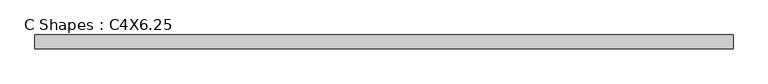
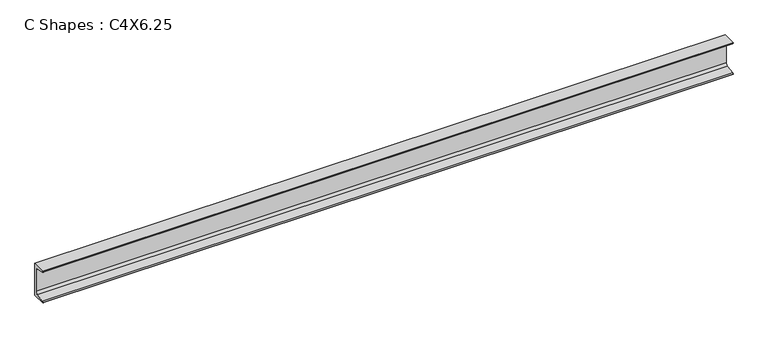
"""IFC4 building model written with IfcOpenShell, lengths in millimetres: beam geometry, C Shapes : C4X6.25."""

from ifc_helpers import new_model, si_unit, point, frame, frame_2d, origin, place, context, project, spatial, polyline, circle_curve, trimmed, segment, composite_curve, outline, extrude, source, transform, mapped, element, save


def c_shapes_c4x6_25_9ff4ea91(model_context):
    return source(origin(), model_context, "Body", "SweptSolid", [
        extrude(outline(composite_curve([segment(polyline([(11.049, 50.8), (11.049, -50.8), (-30.861, -50.8), (-30.861, -49.7865772)]), True, "CONTINUOUS"), segment(trimmed(circle_curve(frame_2d((-27.4066, -49.7865772)), 3.4544), [point((-30.861, -49.7865772))], [point((-27.9743618, -46.379155))], False, "CARTESIAN"), True, "CONTINUOUS"), segment(polyline([(-27.9743618, -46.379155), (-0.9980765, -41.8842311)]), True, "CONTINUOUS"), segment(trimmed(circle_curve(frame_2d((-2.1336, -35.0693868)), 6.9088), [point((-0.9980765, -41.8842311))], [point((4.7752, -35.0693868))], True, "CARTESIAN"), True, "CONTINUOUS"), segment(polyline([(4.7752, -35.0693868), (4.7752, 35.0693868)]), True, "CONTINUOUS"), segment(trimmed(circle_curve(frame_2d((-2.1336, 35.0693868)), 6.9088), [point((4.7752, 35.0693868))], [point((-0.9980765, 41.8842311))], True, "CARTESIAN"), True, "CONTINUOUS"), segment(polyline([(-0.9980765, 41.8842311), (-27.9743618, 46.379155)]), True, "CONTINUOUS"), segment(trimmed(circle_curve(frame_2d((-27.4066, 49.7865772)), 3.4544), [point((-27.9743618, 46.379155))], [point((-30.861, 49.7865772))], False, "CARTESIAN"), True, "CONTINUOUS"), segment(polyline([(-30.861, 49.7865772), (-30.861, 50.8), (11.049, 50.8)]), True, "CONTINUOUS")], self_intersect=False)), frame((-1049.3744237, 0.0, 0.0), z_axis=(1.0, 0.0, 0.0), x_axis=(0.0, 1.0, 0.0)), (0.0, 0.0, 1.0), 2098.7488474),
    ])


if __name__ == "__main__":
    model = new_model("IFC4")
    model_context = context("Model", 3, world=origin())
    ifc_project = project(units=[si_unit("LENGTHUNIT", "METRE", prefix="MILLI")], contexts=[model_context])
    site = spatial("IfcSite", under=ifc_project)
    building = spatial("IfcBuilding", under=site)
    placement = place(None, origin())
    c_shapes_c4x6_25_shape = c_shapes_c4x6_25_9ff4ea91(model_context)
    element("IfcBeam", 1, ObjectType="C Shapes : C4X6.25", at=placement, inside=building, context=model_context, shape_type="MappedRepresentation", body=[
        mapped(c_shapes_c4x6_25_shape, transform((0.0, 0.0, 0.0), x_axis=(1.0, 0.0, 0.0), y_axis=(0.0, 1.0, 0.0), z_axis=(0.0, 0.0, 1.0))),
    ])
    save(model, "model.ifc")

# Revit data of these elements
# Type "C Shapes : C4X6.25"
#   Section Name Key = "ChannelsC4X6.25"
#   Assembly Code = "B10"
#   Width = 1.650"
#   Web Thickness = 0.247"
#   Web Fillet = 0.272"
#   Warping Constant = 1.03 in⁶
#   Torsional Moment of Inertia = 0.0487 in⁴
#   Sloped Flange Angle = 9.46°
#   Section Area = 1.77 in²
#   Plastic Modulus weak axis = 0.569 in³
#   Plastic Modulus strong axis = 2.43 in³
#   Nominal Weight = 6.25 lbf/ft
#   Moment of Inertia weak axis = 0.345 in⁴
#   Moment of Inertia strong axis = 4.00 in⁴
#   Height = 4.000"
#   Flange Thickness Location = 0.7015"
#   Flange Thickness = 0.272"
#   Flange Fillet = 0.136"
#   Elastic Modulus weak axis = 0.284 in³
#   Elastic Modulus strong axis = 2.00 in³
#   Centroid Vertical = 2.000"
#   Centroid Horizontal = 0.435"
#   Length [instance default] = 5' - 0"
#   Structural Material [instance default] = Steel ASTM A36
#   Principal Axes Angle = 0
#   Bolt Spacing = 0
# Element 1 (IfcBeam, "C Shapes : C4X6.25")
#   Materials on its faces: "Steel ASTM A36"
# Materials
#   "Steel ASTM A36": class "Metal", colour RGB 199 199 199, transparency 0, Description = "Structural steel, ASTM A36 Grade B, mill finish", Cost = 0
